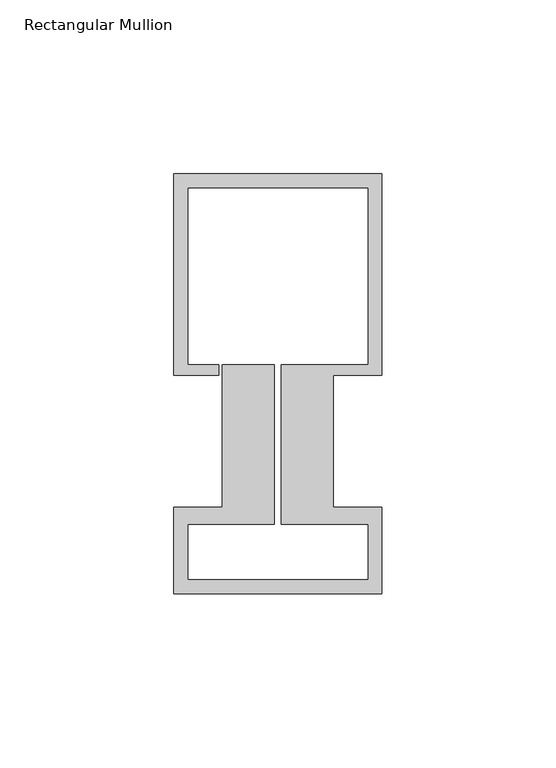
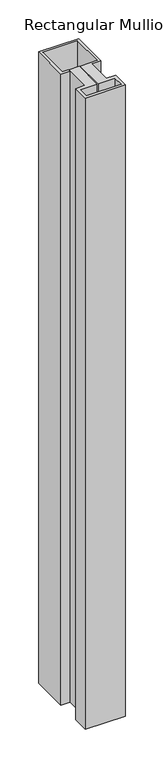
"""IFC4 building model written with IfcOpenShell, lengths in millimetres: member geometry, Rectangular Mullion : Schueco_FWS-60-SI_Tran_CovCap-20mm_Tran-55mm."""

from ifc_helpers import new_model, si_unit, frame, origin, place, context, project, spatial, polyline, outline, extrude, source, transform, mapped, element, save


def rectangular_mullion_653926ae(model_context):
    return source(origin(), model_context, "Body", "SweptSolid", [
        extrude(outline(polyline([(0.0, 96.0), (0.0, 38.0), (-14.0, 38.0), (-14.0, -0.1), (0.0, -0.1), (0.0, -25.0), (-60.0, -25.0), (-60.0, -0.1), (-46.0, -0.1), (-46.0, 41.0), (-31.0, 41.0), (-31.0, -5.0), (-56.0, -5.0), (-56.0, -21.0), (-4.0, -21.0), (-4.0, -5.0), (-29.0, -5.0), (-29.0, 41.0), (-4.0, 41.0), (-4.0, 92.0), (-56.0, 92.0), (-56.0, 41.0), (-47.0, 41.0), (-47.0, 38.0), (-60.0, 38.0), (-60.0, 96.0), (0.0, 96.0)])), frame((0.0, 0.0, -1000.0), z_axis=(0.0, 0.0, 1.0), x_axis=(1.0, 0.0, 0.0)), (0.0, 0.0, 1.0), 1000.0),
    ])


if __name__ == "__main__":
    model = new_model("IFC4")
    model_context = context("Model", 3, world=origin())
    ifc_project = project(units=[si_unit("LENGTHUNIT", "METRE", prefix="MILLI")], contexts=[model_context])
    site = spatial("IfcSite", under=ifc_project)
    building = spatial("IfcBuilding", under=site)
    placement = place(None, origin())
    rectangular_mullion_shape = rectangular_mullion_653926ae(model_context)
    element("IfcMember", 1, ObjectType="Rectangular Mullion : Schueco_FWS-60-SI_Tran_CovCap-20mm_Tran-55mm", at=placement, inside=building, context=model_context, shape_type="MappedRepresentation", body=[
        mapped(rectangular_mullion_shape, transform((0.0, 0.0, 0.0), x_axis=(1.0, 0.0, 0.0), y_axis=(0.0, 1.0, 0.0), z_axis=(0.0, 0.0, 1.0))),
    ])
    save(model, "model.ifc")

# Revit data of these elements
# Type "Rectangular Mullion : Schueco_FWS-60-SI_Tran_CovCap-20mm_Tran-55mm"
#   Model = "FWS 60.SI"
#   Manufacturer = "Schueco International KG"
#   Type Comments = "Transom"
#   Schueco thermal insulation standard = "Suitable for passive houses"
#   Burglar resistance = "RC 3"
#   Thermal insulation = "to 0.70 W/(m²K)"
#   built-in parameter 1007322 = 0.396982 (stored number, unit not read)
#   built-in parameter 1007321 = 0.0524934 (stored number, unit not read)
#   built-in parameter 1007320 = 0.0524934 (stored number, unit not read)
# Element 1 (IfcMember, "Rectangular Mullion : Schueco_FWS-60-SI_Tran_CovCap-20mm_Tran-55mm")
#   Materials on its faces: "Alu"
# Materials
#   "Alu": class "Glas", colour RGB 140 140 140, transparency 0
